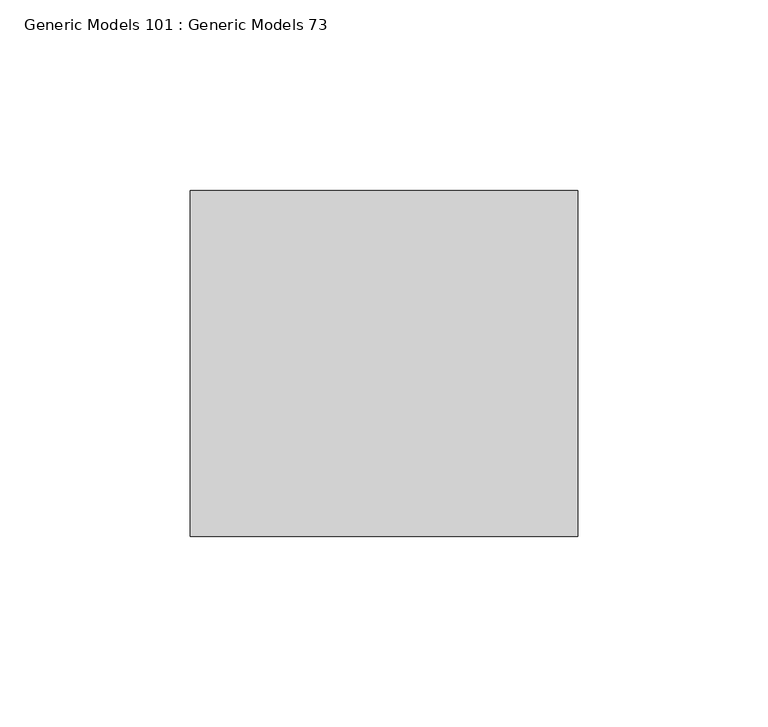
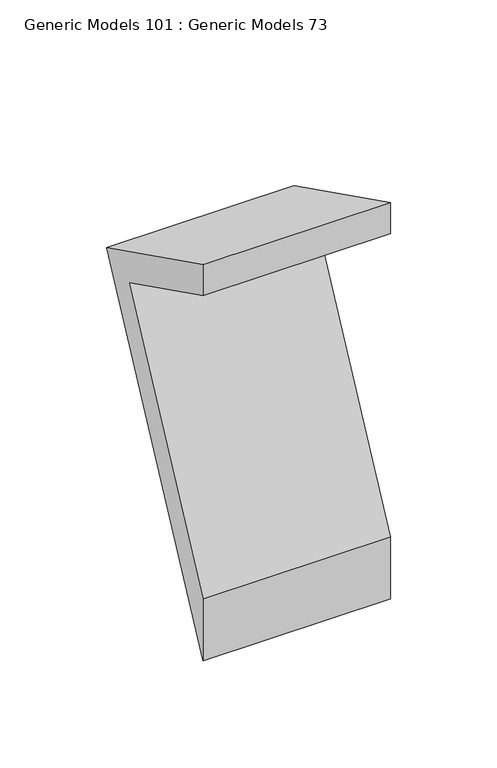
"""IFC4 building model written with IfcOpenShell, lengths in millimetres: proxy geometry, Generic Models 101 : Generic Models 73."""

from ifc_helpers import new_model, si_unit, frame, origin, place, context, project, spatial, polyline, outline, extrude, source, transform, mapped, element, save


def generic_models_101_generic_models_73_6649d40c(model_context):
    return source(origin(), model_context, "Body", "SweptSolid", [
        extrude(outline(polyline([(30949.3519638, 268704.0255987), (30858.4781612, 268522.2779935), (30858.4781612, 268557.7755726), (30928.0534163, 268696.9260829), (30858.4781612, 268731.7137104), (30858.4781612, 268749.4625), (30949.3519638, 268704.0255987)])), frame((31924.6096032, 0.0, 0.0), z_axis=(1.0, 0.0, 0.0), x_axis=(0.0, 1.0, 0.0)), (0.0, 0.0, 1.0), 101.6),
    ])


if __name__ == "__main__":
    model = new_model("IFC4")
    model_context = context("Model", 3, world=origin())
    ifc_project = project(units=[si_unit("LENGTHUNIT", "METRE", prefix="MILLI")], contexts=[model_context])
    site = spatial("IfcSite", under=ifc_project)
    building = spatial("IfcBuilding", under=site)
    placement = place(None, origin())
    generic_models_101_generic_models_73_shape = generic_models_101_generic_models_73_6649d40c(model_context)
    element("IfcBuildingElementProxy", 1, Name="Generic Models 101 : Generic Models 73", ObjectType="Generic Models 101 : Generic Models 73", at=placement, inside=building, context=model_context, shape_type="MappedRepresentation", body=[
        mapped(generic_models_101_generic_models_73_shape, transform((0.0, 0.0, 0.0), x_axis=(1.0, 0.0, 0.0), y_axis=(0.0, 1.0, 0.0), z_axis=(0.0, 0.0, 1.0))),
    ])
    save(model, "model.ifc")

# Revit data of these elements
# Element 1 (IfcBuildingElementProxy, "Generic Models 101 : Generic Models 73")
#   Materials on its faces: "L8 x 4 x 5/8 x 0'-4\" METAL ANGLE"
# Materials
#   "L8 x 4 x 5/8 x 0'-4\" METAL ANGLE": class "Metal", colour RGB 199 199 199, transparency 0, Description = "Carbon steel", Cost = 0
